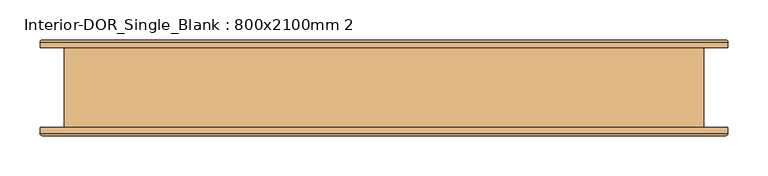
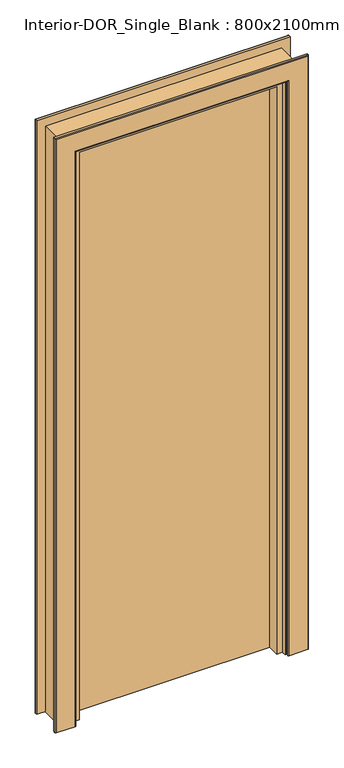
"""IFC4 building model written with IfcOpenShell, lengths in millimetres: door geometry, Interior-DOR_Single_Blank : 800x2100mm 2."""

from ifc_helpers import new_model, si_unit, frame, origin, origin_with_axes, place, context, project, spatial, polyline, circle_curve, ellipse_curve, outline, extrude, faceted_brep, source, transform, mapped, element, save
from ifc_brep_helpers import plane_surface, cylinder_surface, advanced_brep


def interior_dor_single_blank_800x2100mm_2_9dcdbc73(model_context):
    return source(origin(), model_context, "Body", "SolidModel", [
        advanced_brep(
        [(-360.0, 50.0, 0.0), (-430.0, 50.0, 0.0), (-430.0, 57.0, 0.0), (-427.0, 60.0, 0.0), (-363.0, 60.0, 0.0), (-360.0, 57.0, 0.0), (-360.0, 57.0, 2060.0), (-360.0, 50.0, 2060.0), (-363.0, 60.0, 2063.0), (-427.0, 60.0, 2127.0), (427.0, 60.0, 2127.0), (427.0, 60.0, 0.0), (363.0, 60.0, 0.0), (363.0, 60.0, 2063.0), (-430.0, 57.0, 2130.0), (-430.0, 50.0, 2130.0), (360.0, 50.0, 2060.0), (360.0, 50.0, 0.0), (430.0, 50.0, 0.0), (430.0, 50.0, 2130.0), (360.0, 57.0, 0.0), (360.0, 57.0, 2060.0), (430.0, 57.0, 0.0), (430.0, 57.0, 2130.0)],
        [
            (0, 1),
            (1, 2),
            (2, 3, circle_curve(frame((-427.0, 57.0, 0.0), z_axis=(0.0, 0.0, -1.0), x_axis=(-1.0, 0.0, 0.0)), 3.0)),
            (3, 4),
            (4, 5, circle_curve(frame((-363.0, 57.0, 0.0), z_axis=(0.0, 0.0, -1.0), x_axis=(-1.0, 0.0, 0.0)), 3.0)),
            (5, 0),
            (5, 6),
            (6, 7),
            (7, 0),
            (4, 8),
            (8, 6, ellipse_curve(frame((-363.0, 57.0, 2063.0), z_axis=(-0.7071067811865475, 0.0, -0.7071067811865475), x_axis=(0.7071067811865474, 0.0, -0.7071067811865476)), 4.2426407, 3.0)),
            (3, 9),
            (9, 10),
            (10, 11),
            (11, 12),
            (12, 13),
            (13, 8),
            (2, 14),
            (14, 9, ellipse_curve(frame((-427.0, 57.0, 2127.0), z_axis=(-0.7071067811865475, 0.0, -0.7071067811865475), x_axis=(0.7071067811865474, 0.0, -0.7071067811865476)), 4.2426407, 3.0)),
            (1, 15),
            (15, 14),
            (7, 16),
            (16, 17),
            (17, 18),
            (18, 19),
            (19, 15),
            (12, 20, circle_curve(frame((363.0, 57.0, 0.0), z_axis=(0.0, 0.0, 1.0), x_axis=(1.0, 0.0, 0.0)), 3.0)),
            (20, 21),
            (21, 13, ellipse_curve(frame((363.0, 57.0, 2063.0), z_axis=(0.7071067811865475, 0.0, -0.7071067811865475), x_axis=(0.7071067811865474, 0.0, 0.7071067811865476)), 4.2426407, 3.0)),
            (17, 20),
            (11, 22, circle_curve(frame((427.0, 57.0, 0.0), z_axis=(0.0, 0.0, -1.0), x_axis=(1.0, 0.0, 0.0)), 3.0)),
            (22, 18),
            (23, 22),
            (10, 23, ellipse_curve(frame((427.0, 57.0, 2127.0), z_axis=(0.7071067811865475, 0.0, -0.7071067811865475), x_axis=(0.7071067811865474, 0.0, 0.7071067811865476)), 4.2426407, 3.0)),
            (23, 19),
            (16, 21),
            (6, 21),
            (14, 23),
        ],
        [
            plane_surface(frame((-400.0, -50.0, 0.0), z_axis=(0.0, 0.0, -1.0), x_axis=(0.0, 1.0, 0.0))),
            plane_surface(frame((-360.0, 50.0, 0.0), z_axis=(1.0, 0.0, 0.0), x_axis=(0.0, 0.0, 1.0))),
            cylinder_surface(frame((-363.0, 57.0, 0.0), z_axis=(0.0, 0.0, -1.0), x_axis=(-1.0, 0.0, 0.0)), 3.0),
            plane_surface(frame((-363.0, 60.0, 0.0), z_axis=(0.0, 1.0, 0.0), x_axis=(0.0, 0.0, 1.0))),
            cylinder_surface(frame((-427.0, 57.0, 0.0), z_axis=(0.0, 0.0, -1.0), x_axis=(-1.0, 0.0, 0.0)), 3.0),
            plane_surface(frame((-430.0, 57.0, 0.0), z_axis=(-1.0, 0.0, 0.0), x_axis=(0.0, 0.0, 1.0))),
            plane_surface(frame((-430.0, 50.0, 0.0), z_axis=(0.0, -1.0, 0.0), x_axis=(0.0, 0.0, 1.0))),
            cylinder_surface(frame((363.0, 57.0, 2100.0), z_axis=(0.0, 0.0, 1.0), x_axis=(1.0, 0.0, 0.0)), 3.0),
            plane_surface(frame((400.0, -50.0, 0.0), z_axis=(0.0, 0.0, -1.0), x_axis=(0.0, 1.0, 0.0))),
            cylinder_surface(frame((427.0, 57.0, 2100.0), z_axis=(0.0, 0.0, 1.0), x_axis=(1.0, 0.0, 0.0)), 3.0),
            plane_surface(frame((430.0, 57.0, 2130.0), z_axis=(1.0, 0.0, 0.0), x_axis=(0.0, 0.0, -1.0))),
            plane_surface(frame((360.0, 50.0, 2060.0), z_axis=(-1.0, 0.0, 0.0), x_axis=(0.0, 0.0, -1.0))),
            plane_surface(frame((-360.0, 50.0, 2060.0), z_axis=(0.0, 0.0, -1.0), x_axis=(1.0, 0.0, 0.0))),
            cylinder_surface(frame((-400.0, 57.0, 2063.0), z_axis=(-1.0, 0.0, 0.0), x_axis=(0.0, 0.0, 1.0)), 3.0),
            cylinder_surface(frame((-400.0, 57.0, 2127.0), z_axis=(-1.0, 0.0, 0.0), x_axis=(0.0, 0.0, 1.0)), 3.0),
            plane_surface(frame((-430.0, 57.0, 2130.0), z_axis=(0.0, 0.0, 1.0), x_axis=(1.0, 0.0, 0.0))),
        ],
        [
            (0, [[1, 2, 3, 4, 5, 6]]),
            (1, [[7, 8, 9, -6]]),
            (2, [[10, 11, -7, -5]]),
            (3, [[12, 13, 14, 15, 16, 17, -10, -4]]),
            (4, [[18, 19, -12, -3]]),
            (5, [[20, 21, -18, -2]]),
            (6, [[-9, 22, 23, 24, 25, 26, -20, -1]]),
            (7, [[-16, 27, 28, 29]]),
            (8, [[30, -27, -15, 31, 32, -24]]),
            (9, [[33, -31, -14, 34]]),
            (10, [[-25, -32, -33, 35]]),
            (11, [[-28, -30, -23, 36]]),
            (12, [[37, -36, -22, -8]]),
            (13, [[-17, -29, -37, -11]]),
            (14, [[38, -34, -13, -19]]),
            (15, [[-26, -35, -38, -21]]),
        ],
    ),
        advanced_brep(
        [(-430.0, -50.0, 0.0), (-360.0, -50.0, 0.0), (-360.0, -57.0, 0.0), (-363.0, -60.0, 0.0), (-427.0, -60.0, 0.0), (-430.0, -57.0, 0.0), (-430.0, -57.0, 2130.0), (-430.0, -50.0, 2130.0), (-427.0, -60.0, 2127.0), (-363.0, -60.0, 2063.0), (363.0, -60.0, 2063.0), (363.0, -60.0, 0.0), (427.0, -60.0, 0.0), (427.0, -60.0, 2127.0), (-360.0, -57.0, 2060.0), (-360.0, -50.0, 2060.0), (430.0, -50.0, 2130.0), (430.0, -50.0, 0.0), (360.0, -50.0, 0.0), (360.0, -50.0, 2060.0), (430.0, -57.0, 0.0), (430.0, -57.0, 2130.0), (360.0, -57.0, 0.0), (360.0, -57.0, 2060.0)],
        [
            (0, 1),
            (1, 2),
            (2, 3, circle_curve(frame((-363.0, -57.0, 0.0), z_axis=(0.0, 0.0, -1.0), x_axis=(-1.0, 0.0, 0.0)), 3.0)),
            (3, 4),
            (4, 5, circle_curve(frame((-427.0, -57.0, 0.0), z_axis=(0.0, 0.0, -1.0), x_axis=(-1.0, 0.0, 0.0)), 3.0)),
            (5, 0),
            (5, 6),
            (6, 7),
            (7, 0),
            (4, 8),
            (8, 6, ellipse_curve(frame((-427.0, -57.0, 2127.0), z_axis=(-0.7071067811865475, 0.0, -0.7071067811865475), x_axis=(0.7071067811865474, 0.0, -0.7071067811865476)), 4.2426407, 3.0)),
            (3, 9),
            (9, 10),
            (10, 11),
            (11, 12),
            (12, 13),
            (13, 8),
            (2, 14),
            (14, 9, ellipse_curve(frame((-363.0, -57.0, 2063.0), z_axis=(-0.7071067811865475, 0.0, -0.7071067811865475), x_axis=(0.7071067811865474, 0.0, -0.7071067811865476)), 4.2426407, 3.0)),
            (1, 15),
            (15, 14),
            (7, 16),
            (16, 17),
            (17, 18),
            (18, 19),
            (19, 15),
            (12, 20, circle_curve(frame((427.0, -57.0, 0.0), z_axis=(0.0, 0.0, 1.0), x_axis=(1.0, 0.0, 0.0)), 3.0)),
            (20, 21),
            (21, 13, ellipse_curve(frame((427.0, -57.0, 2127.0), z_axis=(0.7071067811865475, 0.0, -0.7071067811865475), x_axis=(0.7071067811865474, 0.0, 0.7071067811865476)), 4.2426407, 3.0)),
            (17, 20),
            (11, 22, circle_curve(frame((363.0, -57.0, 0.0), z_axis=(0.0, 0.0, -1.0), x_axis=(1.0, 0.0, 0.0)), 3.0)),
            (22, 18),
            (23, 22),
            (10, 23, ellipse_curve(frame((363.0, -57.0, 2063.0), z_axis=(0.7071067811865475, 0.0, -0.7071067811865475), x_axis=(0.7071067811865474, 0.0, 0.7071067811865476)), 4.2426407, 3.0)),
            (23, 19),
            (16, 21),
            (6, 21),
            (14, 23),
        ],
        [
            plane_surface(frame((-400.0, -50.0, 0.0), z_axis=(0.0, 0.0, -1.0), x_axis=(0.0, 1.0, 0.0))),
            plane_surface(frame((-430.0, -50.0, 0.0), z_axis=(-1.0, 0.0, 0.0), x_axis=(0.0, 0.0, 1.0))),
            cylinder_surface(frame((-427.0, -57.0, 0.0), z_axis=(0.0, 0.0, -1.0), x_axis=(-1.0, 0.0, 0.0)), 3.0),
            plane_surface(frame((-427.0, -60.0, 0.0), z_axis=(0.0, -1.0, 0.0), x_axis=(0.0, 0.0, 1.0))),
            cylinder_surface(frame((-363.0, -57.0, 0.0), z_axis=(0.0, 0.0, -1.0), x_axis=(-1.0, 0.0, 0.0)), 3.0),
            plane_surface(frame((-360.0, -57.0, 0.0), z_axis=(1.0, 0.0, 0.0), x_axis=(0.0, 0.0, 1.0))),
            plane_surface(frame((-360.0, -50.0, 0.0), z_axis=(0.0, 1.0, 0.0), x_axis=(0.0, 0.0, 1.0))),
            cylinder_surface(frame((427.0, -57.0, 2100.0), z_axis=(0.0, 0.0, 1.0), x_axis=(1.0, 0.0, 0.0)), 3.0),
            plane_surface(frame((400.0, -50.0, 0.0), z_axis=(0.0, 0.0, -1.0), x_axis=(0.0, 1.0, 0.0))),
            cylinder_surface(frame((363.0, -57.0, 2100.0), z_axis=(0.0, 0.0, 1.0), x_axis=(1.0, 0.0, 0.0)), 3.0),
            plane_surface(frame((360.0, -57.0, 2060.0), z_axis=(-1.0, 0.0, 0.0), x_axis=(0.0, 0.0, -1.0))),
            plane_surface(frame((430.0, -50.0, 2130.0), z_axis=(1.0, 0.0, 0.0), x_axis=(0.0, 0.0, -1.0))),
            plane_surface(frame((-430.0, -50.0, 2130.0), z_axis=(0.0, 0.0, 1.0), x_axis=(1.0, 0.0, 0.0))),
            cylinder_surface(frame((-400.0, -57.0, 2127.0), z_axis=(-1.0, 0.0, 0.0), x_axis=(0.0, 0.0, 1.0)), 3.0),
            cylinder_surface(frame((-400.0, -57.0, 2063.0), z_axis=(-1.0, 0.0, 0.0), x_axis=(0.0, 0.0, 1.0)), 3.0),
            plane_surface(frame((-360.0, -57.0, 2060.0), z_axis=(0.0, 0.0, -1.0), x_axis=(1.0, 0.0, 0.0))),
        ],
        [
            (0, [[1, 2, 3, 4, 5, 6]]),
            (1, [[7, 8, 9, -6]]),
            (2, [[10, 11, -7, -5]]),
            (3, [[12, 13, 14, 15, 16, 17, -10, -4]]),
            (4, [[18, 19, -12, -3]]),
            (5, [[20, 21, -18, -2]]),
            (6, [[-9, 22, 23, 24, 25, 26, -20, -1]]),
            (7, [[-16, 27, 28, 29]]),
            (8, [[30, -27, -15, 31, 32, -24]]),
            (9, [[33, -31, -14, 34]]),
            (10, [[-25, -32, -33, 35]]),
            (11, [[-28, -30, -23, 36]]),
            (12, [[37, -36, -22, -8]]),
            (13, [[-17, -29, -37, -11]]),
            (14, [[38, -34, -13, -19]]),
            (15, [[-26, -35, -38, -21]]),
        ],
    ),
        faceted_brep([(-400.0, -50.0, 0.0), (-400.0, 50.0, 0.0), (-355.0, 50.0, 0.0), (-355.0, 5.0, 0.0), (-335.0, 5.0, 0.0), (-335.0, -35.0, 0.0), (-355.0, -35.0, 0.0), (-355.0, -50.0, 0.0), (-355.0, -50.0, 2055.0), (355.0, -50.0, 2055.0), (355.0, -50.0, 0.0), (400.0, -50.0, 0.0), (400.0, -50.0, 2100.0), (-400.0, -50.0, 2100.0), (-355.0, -35.0, 2055.0), (-335.0, -35.0, 2035.0), (335.0, -35.0, 2035.0), (335.0, -35.0, 0.0), (355.0, -35.0, 0.0), (355.0, -35.0, 2055.0), (-335.0, 5.0, 2035.0), (-355.0, 5.0, 2055.0), (355.0, 5.0, 2055.0), (355.0, 5.0, 0.0), (335.0, 5.0, 0.0), (335.0, 5.0, 2035.0), (-355.0, 50.0, 2055.0), (-400.0, 50.0, 2100.0), (400.0, 50.0, 2100.0), (400.0, 50.0, 0.0), (355.0, 50.0, 0.0), (355.0, 50.0, 2055.0)], [[[0, 1, 2, 3, 4, 5, 6, 7]], [[7, 8, 9, 10, 11, 12, 13, 0]], [[6, 14, 8, 7]], [[5, 15, 16, 17, 18, 19, 14, 6]], [[4, 20, 15, 5]], [[3, 21, 22, 23, 24, 25, 20, 4]], [[2, 26, 21, 3]], [[1, 27, 28, 29, 30, 31, 26, 2]], [[0, 13, 27, 1]], [[12, 11, 29, 28]], [[11, 10, 18, 17, 24, 23, 30, 29]], [[19, 18, 10, 9]], [[25, 24, 17, 16]], [[31, 30, 23, 22]], [[20, 25, 16, 15]], [[26, 31, 22, 21]], [[13, 12, 28, 27]], [[14, 19, 9, 8]]]),
        extrude(outline(polyline([(355.0, 50.0), (355.0, 5.0), (-355.0, 5.0), (-355.0, 50.0), (355.0, 50.0)])), origin_with_axes(), (0.0, 0.0, 1.0), 2055.0),
    ])


if __name__ == "__main__":
    model = new_model("IFC4")
    model_context = context("Model", 3, world=origin())
    ifc_project = project(units=[si_unit("LENGTHUNIT", "METRE", prefix="MILLI")], contexts=[model_context])
    site = spatial("IfcSite", under=ifc_project)
    building = spatial("IfcBuilding", under=site)
    placement = place(None, origin())
    interior_dor_single_blank_800x2100mm_2_shape = interior_dor_single_blank_800x2100mm_2_9dcdbc73(model_context)
    element("IfcDoor", 1, ObjectType="Interior-DOR_Single_Blank : 800x2100mm 2", at=placement, inside=building, context=model_context, shape_type="MappedRepresentation", body=[
        mapped(interior_dor_single_blank_800x2100mm_2_shape, transform((0.0, 0.0, 0.0), x_axis=(1.0, 0.0, 0.0), y_axis=(0.0, 1.0, 0.0), z_axis=(0.0, 0.0, 1.0))),
    ])
    save(model, "model.ifc")

# Revit data of these elements
# Type "Interior-DOR_Single_Blank : 800x2100mm 2"
#   Type IfcGUID = "0dwJ1JWsv3L8A_XhzwP5MW"
#   Assembly Code = "C1020120"
#   Type Mark = "195"
#   Classification.Uniclass.EF.Number = "EF_25_30"
#   Classification.Uniclass.EF.Description = "Doors and windows"
#   WindLoadRating = "n/a"
#   WaterTightnessRating = "n/a"
#   WarrantyStartDate [instance default] = "1900-12-31T23:59:59"
#   WarrantyGuarantorParts = "n/a"
#   WarrantyGuarantorLabor = "n/a"
#   WarrantyDurationUnit = "year"
#   WarrantyDurationParts = "n/a"
#   WarrantyDurationLabor = "n/a"
#   WarrantyDescription = "n/a"
#   Version = "2"
#   Uniclass2015Version = "Systems v1.9"
#   Uniclass2015Title = "Doorset systems"
#   Uniclass2015Code = "Ss_25_30_20_25"
#   URL = "www.nationalbimlibrary.com"
#   TagNumber [instance default] = "n/a"
#   SustainabilityPerformance = "n/a"
#   Status = "UNSET"
#   Size = "1010 x 2100 mm"
#   Shape = "n/a"
#   SerialNumber [instance default] = "n/a"
#   SecurityRating = "n/a"
#   Revision = "n/a"
#   ReplacementCost = "n/a"
#   Reference = "n/a"
#   ProductInformation = "n/a"
#   Operation = "SINGLE_SWING_RIGHT"
#   OmniClassVersion = "Table 22 2012-05-16"
#   OmniClassTitle = "Doors and Frames"
#   OmniClassCode = "22-08 10 00"
#   Name = "DoorsetSystem_Interior-Single_Blank"
#   NBSReference = "25-50-20/120"
#   NBSDescription = "Doorset system"
#   NBSCertification = "www.nationalbimlibrary.com/cert/mlf45nxc"
#   ModelReference = "Interior Single Door"
#   ModelNumber = "n/a"
#   Model = "Interior Single Door"
#   MechanicalLoadRating = "n/a"
#   Material = "n/a"
#   ManufacturerURL = "n/a"
#   ManufacturerName = "n/a"
#   Manufacturer = "info@theNBS.com"
#   InstallationDate [instance default] = "1900-12-31T23:59:59"
#   IfcExportType = "DOOR"
#   IfcExportAs = "IfcDoorType"
#   HygrothermalRating = "n/a"
#   Grade = "n/a"
#   FireRating = "n/a"
#   Fire Rating = "n/a"
#   Finish = "n/a"
#   Features = "n/a"
#   ExpectedLife = "n/a"
#   DurationUnit = "n/a"
#   DurabilityRating = "n/a"
#   DoorNumber [instance default] = "n/a"
#   Description = "Generic single interior door"
#   Construction Type = "USERDEFINED"
#   Constituents = "n/a"
#   ComponentNumber [instance default] = "n/a"
#   Color = "n/a"
#   CodePerformance = "n/a"
#   Category = "Ss_25_30_20_25:Doorset systems"
#   BarCode [instance default] = "n/a"
#   BIMObjectName = "NBS_DoorsetSystem_Interior-Single_Blank"
#   Author = "NBS"
#   AssetType = "Fixed"
#   AssetIdentifier [instance default] = "n/a"
#   AcousticRating = "n/a"
#   AccessibilityPerformance = "n/a"
#   Width = 0.8 m
#   WallThickness [instance default] = 0.15 m
#   ThresholdHeight = 0.015 m
#   Thickness = 0.15 m
#   ThermalTransmittance = 0
#   StructuralToleranceJamb = 0 m
#   StructuralToleranceHead = 0 m
#   StructuralOpeningWidth = 0.8 m
#   StructuralOpeningHeight = 2.1 m
#   StopProjection = 0.02 m
#   StopDepth = 0.04 m
#   Rough Width [instance default] = 0.8 m
#   Rough Height [instance default] = 2.1 m
#   RebateDepth = 0.045 m
#   PanelWidth = 0.71 m
#   PanelUndercut = 0 m
#   PanelHeight = 2.055 m
#   PanelDepth = 0.045 m
#   OpeningTolerance = 0 m
#   NominalWidth = 0.8 m
#   NominalLength = 0 m
#   NominalHeight = 2.1 m
#   Infiltration = 0
#   Height = 2.1 m
#   GlazingAreaFraction = 0
#   FrameThickness = 0.045 m
#   FrameSetback [instance default] = 0 m
#   FrameDepth [instance default] = 0.15 m
#   FinishThicknessInternal [instance default] = 0 m
#   FinishThicknessExternal [instance default] = 0 m
#   ClearOpeningWidth = 0.67 m
#   ClearOpeningHeight = 2.035 m
#   CalculatedInteriorVoidDepth [instance default] = 0.3 m
#   ArchitraveWidth = 0.07 m
#   ArchitraveThickness = 0.01 m
#   ArchitraveSetbackFromFrameFace = 0.005 m
#   SmokeStop = no
#   SingleRebate = no
#   SelfClosing = no
#   PlantedStop = yes
#   IsExternal = no
#   HasDrive = no
#   HandicapAccessible = no
#   Wall Closure = 4
#   FireExit = no
#   ArchitraveFrontRequired [instance default] = yes
#   ArchitraveBackRequired [instance default] = yes
#   PanelMaterial = NBS_Concept
#   HardwareFinish = NBS_Concept
#   FrameSectionMaterial = NBS_Concept
#   Function = (empty or 0)
#   Cost = 0
# Element 1 (IfcDoor, "Interior-DOR_Single_Blank : 800x2100mm 2")
#   WallThickness = 0.1 m
#   FrameDepth = 0.1 m
#   Materials on its faces: "NBS_Concept"
# Materials
#   "NBS_Concept": class "Generic", colour RGB 255 255 255, transparency 0, Description = "To be specified", Cost = 0
